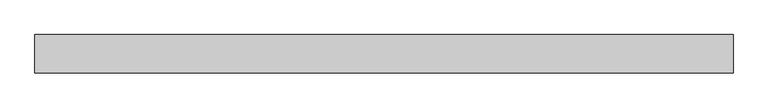
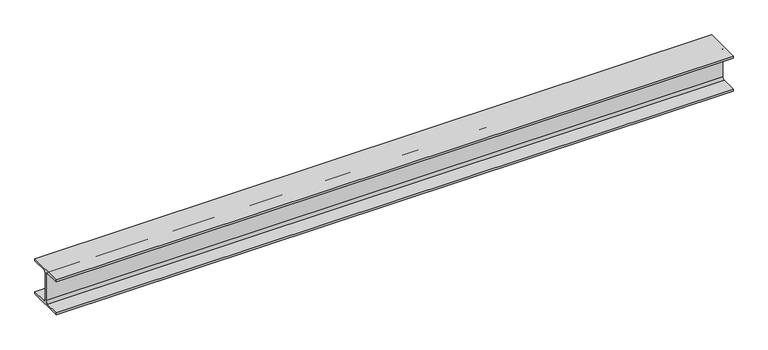
"""IFC4 building model written with IfcOpenShell, lengths in millimetres: beam geometry, 0912_Steel Framing_H-KSD3502 : H_SB_ASB_H-200x200x8x12."""

from ifc_helpers import new_model, si_unit, point, frame, frame_2d, origin, place, context, project, spatial, polyline, circle_curve, trimmed, segment, composite_curve, outline, extrude, source, transform, mapped, element, save


def beam_3ecbfdb4(model_context):
    return source(origin(), model_context, "Body", "SweptSolid", [
        extrude(outline(composite_curve([segment(polyline([(100.0, -88.0), (100.0, -100.0), (-100.0, -100.0), (-100.0, -88.0), (-17.0, -88.0)]), True, "CONTINUOUS"), segment(trimmed(circle_curve(frame_2d((-17.0, -75.0)), 13.0), [point((-17.0, -88.0))], [point((-4.0, -75.0))], True, "CARTESIAN"), True, "CONTINUOUS"), segment(polyline([(-4.0, -75.0), (-4.0, 75.0)]), True, "CONTINUOUS"), segment(trimmed(circle_curve(frame_2d((-17.0, 75.0)), 13.0), [point((-4.0, 75.0))], [point((-17.0, 88.0))], True, "CARTESIAN"), True, "CONTINUOUS"), segment(polyline([(-17.0, 88.0), (-100.0, 88.0), (-100.0, 100.0), (100.0, 100.0), (100.0, 88.0), (17.0, 88.0)]), True, "CONTINUOUS"), segment(trimmed(circle_curve(frame_2d((17.0, 75.0)), 13.0), [point((17.0, 88.0))], [point((4.0, 75.0))], True, "CARTESIAN"), True, "CONTINUOUS"), segment(polyline([(4.0, 75.0), (4.0, -75.0)]), True, "CONTINUOUS"), segment(trimmed(circle_curve(frame_2d((17.0, -75.0)), 13.0), [point((4.0, -75.0))], [point((17.0, -88.0))], True, "CARTESIAN"), True, "CONTINUOUS"), segment(polyline([(17.0, -88.0), (100.0, -88.0)]), True, "CONTINUOUS")], self_intersect=False)), frame((-1914.9296967, 0.0, 0.0), z_axis=(1.0, 0.0, 0.0), x_axis=(0.0, 1.0, 0.0)), (0.0, 0.0, 1.0), 3642.6434861),
    ])


if __name__ == "__main__":
    model = new_model("IFC4")
    model_context = context("Model", 3, world=origin())
    ifc_project = project(units=[si_unit("LENGTHUNIT", "METRE", prefix="MILLI")], contexts=[model_context])
    site = spatial("IfcSite", under=ifc_project)
    building = spatial("IfcBuilding", under=site)
    placement = place(None, origin())
    beam_shape = beam_3ecbfdb4(model_context)
    element("IfcBeam", 1, ObjectType="0912_Steel Framing_H-KSD3502 : H_SB_ASB_H-200x200x8x12", at=placement, inside=building, context=model_context, shape_type="MappedRepresentation", body=[
        mapped(beam_shape, transform((0.0, 0.0, 0.0), x_axis=(1.0, 0.0, 0.0), y_axis=(0.0, 1.0, 0.0), z_axis=(0.0, 0.0, 1.0))),
    ])
    save(model, "model.ifc")

# Revit data of these elements
# Type "0912_Steel Framing_H-KSD3502 : H_SB_ASB_H-200x200x8x12"
#   H_WM Code_1 = "S01AA002-00001 | Main Steel Structure Fabrication Work | Shelter/Building | Medium Steel - Standard (90KG/M>Weight≥30KG/M) | Material: (   )"
#   H_WM Code_2 = "S03AA028-00001 | Main Steel Structure Erection Work | Shelter/Building | Medium Steel (90KG/M>Weight≥30KG/M) | Material: (   )"
#   H_WM Code_3 = "S01AA010-00001 | Main Steel Structure Fabrication Work | Shelter/Building | Steel Painting/Coating | for Non-Fireproofed Steel Surface, Surface Preparation, Primer, Second & Final Coat | Material: (   )"
#   H_Q'ty Cal Type Tag = "SB-Q2"
#   Width = 20.0 cm
#   Web Thickness = 0.8 cm
#   Web Fillet = 1.3 cm
#   Warping Constant = 141000.0 cm⁶
#   W = 0
#   Torsional Moment of Inertia = 26.2485 cm⁴
#   Section Area = 63.53 cm²
#   Plastic Modulus weak axis = 244.0 cm³
#   Plastic Modulus strong axis = 525.0 cm³
#   Perimeter = 1.16 m²/m
#   Nominal Weight = 49.90 kgf/m
#   Moment of Inertia weak axis = 1600.00 cm⁴
#   Moment of Inertia strong axis = 4720.00 cm⁴
#   Height = 20.0 cm
#   Flange Thickness = 1.2 cm
#   Elastic Modulus weak axis = 160.0 cm³
#   Elastic Modulus strong axis = 472.0 cm³
#   Centroid Vertical = 10.0 cm
#   Centroid Horizontal = 10.0 cm
#   Ix = 47200000
#   Length [instance default] = 1.5240 m
#   Zx = 525000
#   b = 0.2000 m
#   h = 0.2000 m
#   r = 0.0130 m
#   s = 0.0080 m
#   t = 0.0120 m
#   A = 0.006353 m²
#   Structural Material [instance default] = Steel, 45-345
#   Assembly Code = ""
# Element 1 (IfcBeam, "0912_Steel Framing_H-KSD3502 : H_SB_ASB_H-200x200x8x12")
#   Structural Material = none
# Materials
#   "Steel, 45-345": class "Metal", colour RGB 189 187 185, transparency 0, Description = "Steel 345 MPa", Cost = 0
